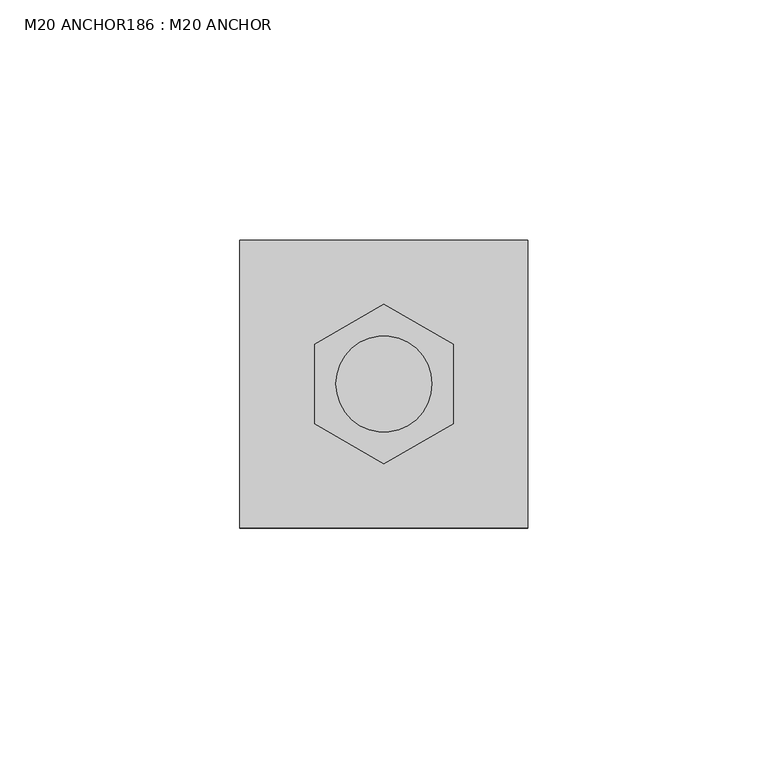
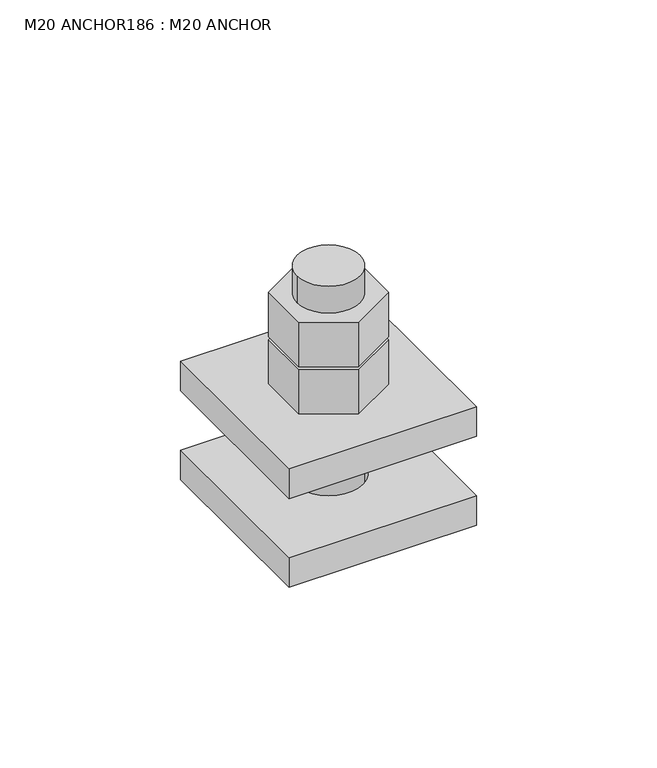
"""IFC4 building model written with IfcOpenShell, lengths in millimetres: fastener geometry, M20 ANCHOR186 : M20 ANCHOR."""

import ifcopenshell
import ifcopenshell.guid

model = None  # the IFC model being written
_history = None  # IfcOwnerHistory: only IFC2X3 demands one
_inside = {}  # id of a spatial element -> (the spatial element, [elements in it])
_under = {}  # id of a project, library or spatial element -> (it, [spatial elements below it])
_declared = {}  # id of a project -> (the project, [libraries it declares])
_typed = {}  # id of a type object -> (the type object, [elements of that type])
_made_of = {}  # id of a material, layer set ... -> (it, [elements and type objects made of it])


def new_model(schema):
    """Start an empty IFC model of exactly this schema.

    Asked for "IFC4X3", IfcOpenShell would pick the latest addendum, in which some entities
    have other attributes; the version numbers below select the first issue.
    IFC2X3 requires an IfcOwnerHistory on every rooted entity: one is made here for all.
    """
    global model, _history
    if schema == "IFC4X3":
        model = ifcopenshell.file(schema_version=(4, 3, 0, 0))
    else:
        model = ifcopenshell.file(schema=schema)
    _inside.clear()
    _under.clear()
    _declared.clear()
    _typed.clear()
    _made_of.clear()
    _history = None
    if model.schema == "IFC2X3":
        org = make("IfcOrganization", Name="unknown")
        user = make(
            "IfcPersonAndOrganization",
            ThePerson=make("IfcPerson", FamilyName="unknown"),
            TheOrganization=org,
        )
        app = make(
            "IfcApplication",
            ApplicationDeveloper=org,
            Version="unknown",
            ApplicationFullName="unknown",
            ApplicationIdentifier="unknown",
        )
        _history = make(
            "IfcOwnerHistory",
            OwningUser=user,
            OwningApplication=app,
            ChangeAction="ADDED",
            CreationDate=0,
        )
    return model


def make(cls, **values):
    """One entity of the class cls with the attributes given. An attribute that is None is left unset."""
    return model.create_entity(
        cls, **{name: value for name, value in values.items() if value is not None}
    )


def rooted(cls, **values):
    """An entity with a GlobalId (a new one), such as an element, a storey or a relation."""
    return make(cls, GlobalId=ifcopenshell.guid.new(), OwnerHistory=_history, **values)


def si_unit(unit_type, name, prefix=None):
    """IfcSIUnit, for example si_unit("LENGTHUNIT", "METRE", prefix="MILLI")."""
    return make("IfcSIUnit", UnitType=unit_type, Prefix=prefix, Name=name)


def assignment(units):
    """IfcUnitAssignment: the units of a project."""
    return None if units is None else make("IfcUnitAssignment", Units=units)


def point(xyz):
    """IfcCartesianPoint."""
    return None if xyz is None else make("IfcCartesianPoint", Coordinates=xyz)


def direction(xyz):
    """IfcDirection."""
    return None if xyz is None else make("IfcDirection", DirectionRatios=xyz)


def frame(location, z_axis=None, x_axis=None):
    """IfcAxis2Placement3D, a coordinate frame: its origin and axes. An axis left out is left unset."""
    return make(
        "IfcAxis2Placement3D",
        Location=point(location),
        Axis=direction(z_axis),
        RefDirection=direction(x_axis),
    )


def frame_2d(location, x_axis=None):
    """IfcAxis2Placement2D, a coordinate frame in the plane: its origin and x axis."""
    return make(
        "IfcAxis2Placement2D", Location=point(location), RefDirection=direction(x_axis)
    )


def origin():
    """The frame at (0, 0, 0) with its axes left unset."""
    return frame((0.0, 0.0, 0.0))


def place(relative_to, where):
    """IfcLocalPlacement: puts the frame where relative to a parent placement (None: the world)."""
    return make(
        "IfcLocalPlacement", PlacementRelTo=relative_to, RelativePlacement=where
    )


def context(
    kind, dimensions, precision=None, world=None, true_north=None, identifier=None
):
    """IfcGeometricRepresentationContext, for example the 3D "Model" context."""
    return make(
        "IfcGeometricRepresentationContext",
        ContextIdentifier=identifier,
        ContextType=kind,
        CoordinateSpaceDimension=dimensions,
        Precision=precision,
        WorldCoordinateSystem=world,
        TrueNorth=true_north,
    )


def project(units=None, contexts=None):
    """IfcProject with its units and contexts."""
    return rooted(
        "IfcProject",
        Name="project",
        RepresentationContexts=contexts,
        UnitsInContext=assignment(units),
    )


def spatial(cls, under=None, at=None, **own):
    """A site, building, storey or space (cls), placed at a placement, below another one or the project."""
    s = rooted(cls, ObjectPlacement=at, **own)
    if under is not None:
        _under.setdefault(under.id(), (under, []))[1].append(s)
    return s


def polyline(points):
    """IfcPolyline through the points."""
    return make("IfcPolyline", Points=[point(p) for p in points])


def circle_curve(where, radius):
    """IfcCircle in the frame where."""
    return make("IfcCircle", Position=where, Radius=radius)


def trimmed(basis, trim1, trim2, sense, master):
    """IfcTrimmedCurve: the piece of a basis curve between two trims."""
    return make(
        "IfcTrimmedCurve",
        BasisCurve=basis,
        Trim1=trim1,
        Trim2=trim2,
        SenseAgreement=sense,
        MasterRepresentation=master,
    )


def segment(curve, same_sense, transition):
    """IfcCompositeCurveSegment."""
    return make(
        "IfcCompositeCurveSegment",
        Transition=transition,
        SameSense=same_sense,
        ParentCurve=curve,
    )


def composite_curve(segments, self_intersect=None):
    """IfcCompositeCurve: segments joined end to end."""
    return make("IfcCompositeCurve", Segments=segments, SelfIntersect=self_intersect)


def outline(outer, holes=None, kind="AREA"):
    """IfcArbitraryClosedProfileDef: a profile drawn as a closed curve; with holes, ...WithVoids."""
    if holes is None:
        return make("IfcArbitraryClosedProfileDef", ProfileType=kind, OuterCurve=outer)
    return make(
        "IfcArbitraryProfileDefWithVoids",
        ProfileType=kind,
        OuterCurve=outer,
        InnerCurves=holes,
    )


def extrude(swept, where, along, depth):
    """IfcExtrudedAreaSolid: the profile swept, set in the frame where, extruded along a direction by depth."""
    return make(
        "IfcExtrudedAreaSolid",
        SweptArea=swept,
        Position=where,
        ExtrudedDirection=direction(along),
        Depth=depth,
    )


def shape(context_of_items, identifier, shape_type, items):
    """IfcShapeRepresentation: the items that make up one representation, for example the "Body"."""
    return make(
        "IfcShapeRepresentation",
        ContextOfItems=context_of_items,
        RepresentationIdentifier=identifier,
        RepresentationType=shape_type,
        Items=items,
    )


def source(mapping_origin, context_of_items, identifier, shape_type, items):
    """IfcRepresentationMap: a shape defined once, which mapped items show again and again."""
    return make(
        "IfcRepresentationMap",
        MappingOrigin=mapping_origin,
        MappedRepresentation=shape(context_of_items, identifier, shape_type, items),
    )


def transform(
    local_origin,
    x_axis=None,
    y_axis=None,
    z_axis=None,
    scale=None,
    scale2=None,
    scale3=None,
    uniform=True,
):
    """IfcCartesianTransformationOperator3D, or its non-uniform kind. x_axis, y_axis, z_axis: its Axis1, 2, 3."""
    if uniform:
        return make(
            "IfcCartesianTransformationOperator3D",
            Axis1=direction(x_axis),
            Axis2=direction(y_axis),
            LocalOrigin=point(local_origin),
            Scale=scale,
            Axis3=direction(z_axis),
        )
    return make(
        "IfcCartesianTransformationOperator3DnonUniform",
        Axis1=direction(x_axis),
        Axis2=direction(y_axis),
        LocalOrigin=point(local_origin),
        Scale=scale,
        Axis3=direction(z_axis),
        Scale2=scale2,
        Scale3=scale3,
    )


def mapped(mapping_source, mapping_target):
    """IfcMappedItem: shows the shape of a source again, moved by a transform."""
    return make(
        "IfcMappedItem", MappingSource=mapping_source, MappingTarget=mapping_target
    )


def made_of(thing, what):
    """Note that an element or type object is made of a material, layer set ...; save() writes the relation."""
    if what is not None:
        _made_of.setdefault(what.id(), (what, []))[1].append(thing)
    return thing


def element(
    cls,
    number,
    at=None,
    inside=None,
    cuts=None,
    type_object=None,
    material=None,
    context=None,
    identifier="Body",
    shape_type=None,
    held_by="IfcProductDefinitionShape",
    body=None,
    shapes=None,
    **own,
):
    """One element of the class cls, such as IfcWall. Its Tag is "e" and its number.

    at: its placement. inside: the storey or other place that contains it. cuts: it is an
    opening in that element (IfcRelVoidsElement). A single representation is given by context,
    identifier, shape_type and body (its items); several are given by shapes. held_by: the class
    of the entity that holds the representations. save() writes the other relations.
    """
    e = rooted(cls, Tag="e%d" % number, ObjectPlacement=at, **own)
    if body is not None:
        shapes = [shape(context, identifier, shape_type, body)]
    if shapes is not None:
        e.Representation = make(held_by, Representations=shapes)
    if inside is not None:
        _inside.setdefault(inside.id(), (inside, []))[1].append(e)
    if cuts is not None:
        rooted(
            "IfcRelVoidsElement", RelatingBuildingElement=cuts, RelatedOpeningElement=e
        )
    if type_object is not None:
        _typed.setdefault(type_object.id(), (type_object, []))[1].append(e)
    return made_of(e, material)


def aggregate(whole, parts):
    """IfcRelAggregates: a whole, such as a stair, and the parts it consists of."""
    return rooted("IfcRelAggregates", RelatingObject=whole, RelatedObjects=parts)


def save(model, path):
    """Write the relations noted so far, then the file.

    IfcRelAggregates (storeys below a building ...), IfcRelContainedInSpatialStructure (elements
    in a storey), IfcRelDefinesByType, IfcRelAssociatesMaterial and IfcRelDeclares: one each for
    every whole, place, type object, material and project.
    """
    for whole, parts in _under.values():
        aggregate(whole, parts)
    for where, things in _inside.values():
        rooted(
            "IfcRelContainedInSpatialStructure",
            RelatedElements=things,
            RelatingStructure=where,
        )
    for kind, things in _typed.values():
        rooted("IfcRelDefinesByType", RelatedObjects=things, RelatingType=kind)
    for what, things in _made_of.values():
        rooted("IfcRelAssociatesMaterial", RelatedObjects=things, RelatingMaterial=what)
    for by, libraries in _declared.values():
        rooted("IfcRelDeclares", RelatingContext=by, RelatedDefinitions=libraries)
    model.write(path)


def m20_anchor186_m20_anchor_bf4e8567(model_context):
    return source(origin(), model_context, "Body", "SweptSolid", [
        extrude(outline(polyline([(6008.0855968, 22545.0952779), (6022.4937158, 22553.4138093), (6036.9018348, 22545.0952779), (6036.9018348, 22528.4582151), (6022.4937158, 22520.1396837), (6008.0855968, 22528.4582151), (6008.0855968, 22545.0952779)]), holes=[composite_curve([segment(trimmed(circle_curve(frame_2d((6022.4937158, 22536.7767465)), 10.0), [point((6032.4937158, 22536.7767465))], [point((6012.4937158, 22536.7767465))], True, "CARTESIAN"), True, "CONTINUOUS"), segment(trimmed(circle_curve(frame_2d((6022.4937158, 22536.7767465)), 10.0), [point((6012.4937158, 22536.7767465))], [point((6032.4937158, 22536.7767465))], True, "CARTESIAN"), True, "CONTINUOUS")], self_intersect=False)]), frame((0.0, 0.0, 246.0), z_axis=(0.0, 0.0, 1.0), x_axis=(1.0, 0.0, 0.0)), (0.0, 0.0, 1.0), 15.0),
        extrude(outline(polyline([(6008.0855968, 22545.0952779), (6022.4937158, 22553.4138093), (6036.9018348, 22545.0952779), (6036.9018348, 22528.4582151), (6022.4937158, 22520.1396837), (6008.0855968, 22528.4582151), (6008.0855968, 22545.0952779)]), holes=[composite_curve([segment(trimmed(circle_curve(frame_2d((6022.4937158, 22536.7767465)), 10.0), [point((6032.4937158, 22536.7767465))], [point((6012.4937158, 22536.7767465))], True, "CARTESIAN"), True, "CONTINUOUS"), segment(trimmed(circle_curve(frame_2d((6022.4937158, 22536.7767465)), 10.0), [point((6012.4937158, 22536.7767465))], [point((6032.4937158, 22536.7767465))], True, "CARTESIAN"), True, "CONTINUOUS")], self_intersect=False)]), frame((0.0, 0.0, 230.0), z_axis=(0.0, 0.0, 1.0), x_axis=(1.0, 0.0, 0.0)), (0.0, 0.0, 1.0), 15.0),
        extrude(outline(composite_curve([segment(trimmed(circle_curve(frame_2d((6022.4937158, 22536.7767465)), 10.0), [point((6032.4937158, 22536.7767465))], [point((6012.4937158, 22536.7767465))], False, "CARTESIAN"), True, "CONTINUOUS"), segment(trimmed(circle_curve(frame_2d((6022.4937158, 22536.7767465)), 10.0), [point((6012.4937158, 22536.7767465))], [point((6032.4937158, 22536.7767465))], False, "CARTESIAN"), True, "CONTINUOUS")], self_intersect=False)), frame((0.0, 0.0, 190.0), z_axis=(0.0, 0.0, 1.0), x_axis=(1.0, 0.0, 0.0)), (0.0, 0.0, 1.0), 80.0),
        extrude(outline(polyline([(5992.4937158, 22566.7767465), (6052.4937158, 22566.7767465), (6052.4937158, 22506.7767465), (5992.4937158, 22506.7767465), (5992.4937158, 22566.7767465)]), holes=[composite_curve([segment(trimmed(circle_curve(frame_2d((6022.4937158, 22536.7767465)), 11.0), [point((6033.4937158, 22536.7767465))], [point((6011.4937158, 22536.7767465))], True, "CARTESIAN"), True, "CONTINUOUS"), segment(trimmed(circle_curve(frame_2d((6022.4937158, 22536.7767465)), 11.0), [point((6011.4937158, 22536.7767465))], [point((6033.4937158, 22536.7767465))], True, "CARTESIAN"), True, "CONTINUOUS")], self_intersect=False)]), frame((0.0, 0.0, 190.0), z_axis=(0.0, 0.0, 1.0), x_axis=(1.0, 0.0, 0.0)), (0.0, 0.0, 1.0), 10.0),
        extrude(outline(polyline([(5992.4937158, 22566.7767465), (6052.4937158, 22566.7767465), (6052.4937158, 22506.7767465), (5992.4937158, 22506.7767465), (5992.4937158, 22566.7767465)]), holes=[composite_curve([segment(trimmed(circle_curve(frame_2d((6022.4937158, 22536.7767465)), 11.0), [point((6033.4937158, 22536.7767465))], [point((6011.4937158, 22536.7767465))], True, "CARTESIAN"), True, "CONTINUOUS"), segment(trimmed(circle_curve(frame_2d((6022.4937158, 22536.7767465)), 11.0), [point((6011.4937158, 22536.7767465))], [point((6033.4937158, 22536.7767465))], True, "CARTESIAN"), True, "CONTINUOUS")], self_intersect=False)]), frame((0.0, 0.0, 220.0), z_axis=(0.0, 0.0, 1.0), x_axis=(1.0, 0.0, 0.0)), (0.0, 0.0, 1.0), 10.0),
    ])


if __name__ == "__main__":
    model = new_model("IFC4")
    model_context = context("Model", 3, world=origin())
    ifc_project = project(units=[si_unit("LENGTHUNIT", "METRE", prefix="MILLI")], contexts=[model_context])
    site = spatial("IfcSite", under=ifc_project)
    building = spatial("IfcBuilding", under=site)
    placement = place(None, origin())
    m20_anchor186_m20_anchor_shape = m20_anchor186_m20_anchor_bf4e8567(model_context)
    element("IfcFastener", 1, ObjectType="M20 ANCHOR186 : M20 ANCHOR", at=placement, inside=building, context=model_context, shape_type="MappedRepresentation", body=[
        mapped(m20_anchor186_m20_anchor_shape, transform((0.0, 0.0, 0.0), x_axis=(1.0, 0.0, 0.0), y_axis=(0.0, 1.0, 0.0), z_axis=(0.0, 0.0, 1.0))),
    ])
    save(model, "model.ifc")
